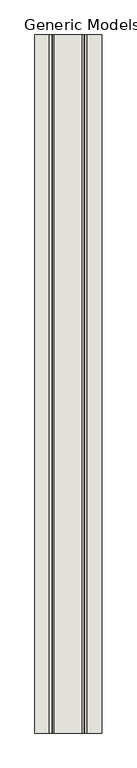
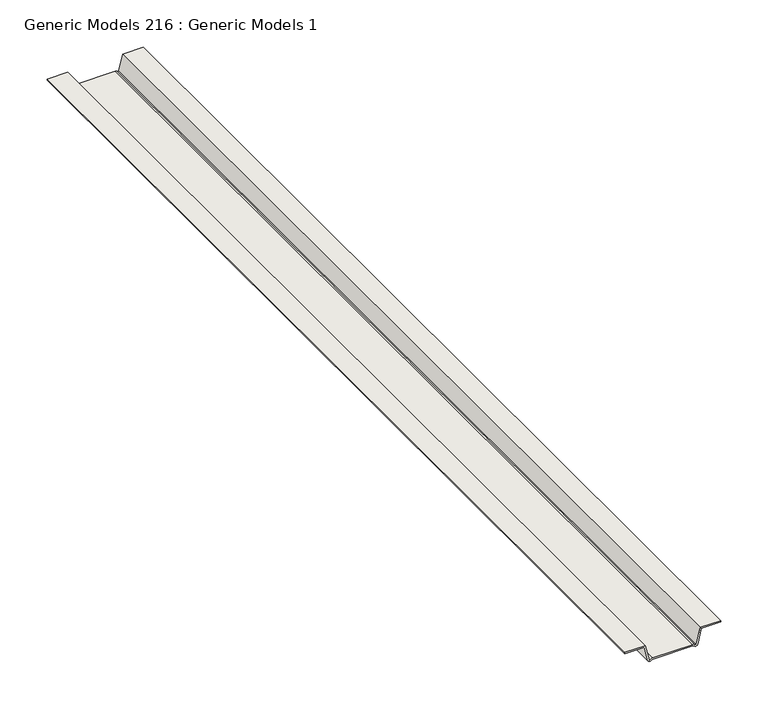
"""IFC4 building model written with IfcOpenShell, lengths in millimetres: wall geometry, Generic Models 216 : Generic Models 1."""

from ifc_helpers import new_model, si_unit, point, frame, frame_2d, origin, place, context, project, spatial, polyline, circle_curve, trimmed, segment, composite_curve, outline, extrude, source, transform, mapped, element, save


def generic_models_216_generic_models_1_d75e17fc(model_context):
    return source(origin(), model_context, "Body", "SweptSolid", [
        extrude(outline(composite_curve([segment(polyline([(7939.0875, 44283.5380487), (7939.0875, 44307.3166382), (7940.675, 44307.3166382), (7940.675, 44282.2625344), (7920.6602886, 44277.8480659)]), True, "CONTINUOUS"), segment(trimmed(circle_curve(frame_2d((7920.83125, 44277.0729458)), 0.79375), [point((7920.6602886, 44277.8480659))], [point((7920.3020833, 44276.4813195))], True, "CARTESIAN"), True, "CONTINUOUS"), segment(trimmed(circle_curve(frame_2d((7917.65625, 44273.5231879)), 3.96875), [point((7920.3020833, 44276.4813195))], [point((7921.625, 44273.5231879))], False, "CARTESIAN"), True, "CONTINUOUS"), segment(polyline([(7921.625, 44273.5231879), (7921.625, 44224.4346459)]), True, "CONTINUOUS"), segment(trimmed(circle_curve(frame_2d((7917.65625, 44224.4346459)), 3.96875), [point((7921.625, 44224.4346459))], [point((7920.3020833, 44221.4765143))], False, "CARTESIAN"), True, "CONTINUOUS"), segment(trimmed(circle_curve(frame_2d((7920.83125, 44220.884888)), 0.79375), [point((7920.3020833, 44221.4765143))], [point((7920.6602886, 44220.1097678))], True, "CARTESIAN"), True, "CONTINUOUS"), segment(polyline([(7920.6602886, 44220.1097678), (7940.675, 44215.6952994), (7940.675, 44190.6411955), (7939.0875, 44190.6411955), (7939.0875, 44214.419785), (7920.3183657, 44218.5595275)]), True, "CONTINUOUS"), segment(trimmed(circle_curve(frame_2d((7920.83125, 44220.884888)), 2.38125), [point((7920.3183657, 44218.5595275))], [point((7919.24375, 44222.6597669))], False, "CARTESIAN"), True, "CONTINUOUS"), segment(trimmed(circle_curve(frame_2d((7917.65625, 44224.4346459)), 2.38125), [point((7919.24375, 44222.6597669))], [point((7920.0375, 44224.4346459))], True, "CARTESIAN"), True, "CONTINUOUS"), segment(polyline([(7920.0375, 44224.4346459), (7920.0375, 44273.5231879)]), True, "CONTINUOUS"), segment(trimmed(circle_curve(frame_2d((7917.65625, 44273.5231879)), 2.38125), [point((7920.0375, 44273.5231879))], [point((7919.24375, 44275.2980668))], True, "CARTESIAN"), True, "CONTINUOUS"), segment(trimmed(circle_curve(frame_2d((7920.83125, 44277.0729458)), 2.38125), [point((7919.24375, 44275.2980668))], [point((7920.3183657, 44279.3983062))], False, "CARTESIAN"), True, "CONTINUOUS"), segment(polyline([(7920.3183657, 44279.3983062), (7939.0875, 44283.5380487)]), True, "CONTINUOUS")], self_intersect=False)), frame((0.0, 0.0, 0.0), z_axis=(0.0, 1.0, 0.0), x_axis=(0.0, 0.0, 1.0)), (0.0, 0.0, 1.0), 1219.2),
    ])


if __name__ == "__main__":
    model = new_model("IFC4")
    model_context = context("Model", 3, world=origin())
    ifc_project = project(units=[si_unit("LENGTHUNIT", "METRE", prefix="MILLI")], contexts=[model_context])
    site = spatial("IfcSite", under=ifc_project)
    building = spatial("IfcBuilding", under=site)
    placement = place(None, origin())
    generic_models_216_generic_models_1_shape = generic_models_216_generic_models_1_d75e17fc(model_context)
    element("IfcWall", 1, ObjectType="Generic Models 216 : Generic Models 1", at=placement, inside=building, context=model_context, shape_type="MappedRepresentation", body=[
        mapped(generic_models_216_generic_models_1_shape, transform((0.0, 0.0, 0.0), x_axis=(1.0, 0.0, 0.0), y_axis=(0.0, 1.0, 0.0), z_axis=(0.0, 0.0, 1.0))),
    ])
    save(model, "model.ifc")

# Revit data of these elements
# Element 1 (IfcWall, "Generic Models 216 : Generic Models 1")
#   Materials on its faces: "7/8\" FURRING CHANNELS @ 16\" O.C."
# Materials
#   "7/8\" FURRING CHANNELS @ 16\" O.C.": class "Unassigned", colour RGB 166 164 162, transparency 0, Keynote = "M05121300.02", Cost = 0
